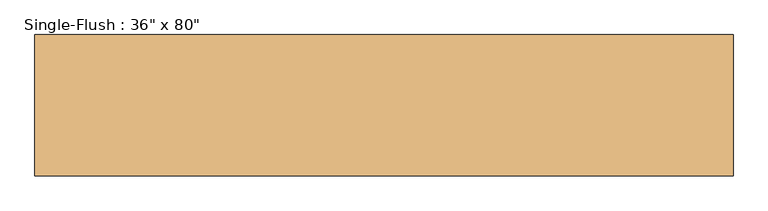
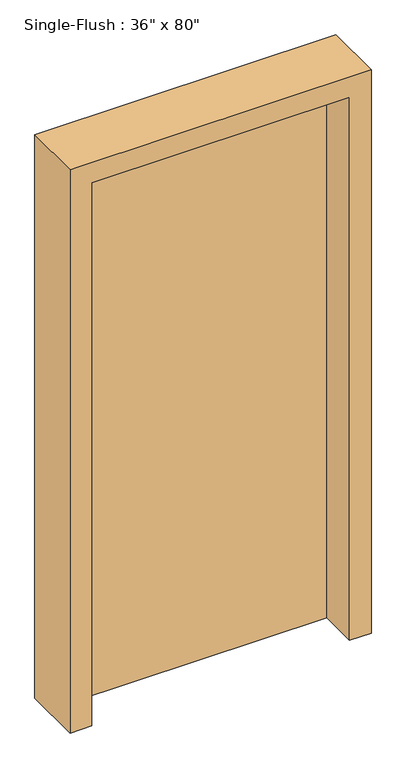
"""IFC4 building model written with IfcOpenShell, lengths in millimetres: door geometry."""

from ifc_helpers import new_model, si_unit, frame, origin, origin_with_axes, place, context, project, spatial, polyline, outline, extrude, source, transform, mapped, element, save


def door_514697dd(model_context):
    return source(origin(), model_context, "Body", "SweptSolid", [
        extrude(outline(polyline([(2108.2, 533.4), (2108.2, -533.4), (0.0, -533.4), (0.0, -457.2), (2032.0, -457.2), (2032.0, 457.2), (0.0, 457.2), (0.0, 533.4), (2108.2, 533.4)])), frame((0.0, -107.95, 0.0), z_axis=(0.0, 1.0, 0.0), x_axis=(0.0, 0.0, 1.0)), (0.0, 0.0, 1.0), 215.9),
        extrude(outline(polyline([(457.2, 31.75), (-457.2, 31.75), (-457.2, 82.55), (457.2, 82.55), (457.2, 31.75)])), origin_with_axes(), (0.0, 0.0, 1.0), 2032.0),
    ])


if __name__ == "__main__":
    model = new_model("IFC4")
    model_context = context("Model", 3, world=origin())
    ifc_project = project(units=[si_unit("LENGTHUNIT", "METRE", prefix="MILLI")], contexts=[model_context])
    site = spatial("IfcSite", under=ifc_project)
    building = spatial("IfcBuilding", under=site)
    placement = place(None, origin())
    door_shape = door_514697dd(model_context)
    element("IfcDoor", 1, ObjectType="Single-Flush : 36\" x 80\"", at=placement, inside=building, context=model_context, shape_type="MappedRepresentation", body=[
        mapped(door_shape, transform((0.0, 0.0, 0.0), x_axis=(1.0, 0.0, 0.0), y_axis=(0.0, 1.0, 0.0), z_axis=(0.0, 0.0, 1.0))),
    ])
    save(model, "model.ifc")

# Revit data of these elements
# Type "Single-Flush : 36\" x 80\""
#   Type Mark = "6"
#   OD_DS_Door_Material = "T.B.D."
#   OD_DS_Door_Type = "SWING"
#   OD_DS_Lockset = "PRIVACY LOCK"
#   Assembly Code = "C1020"
#   Analytic Construction = "<None>"
#   Thickness = 0' - 2"
#   RO Offset = 0' - 0 1/4"
#   Height = 6' - 8"
#   Trim Projection Ext = 0' - 1"
#   Trim Projection Int = 0' - 1"
#   Trim Width = 0' - 3"
#   Width = 3' - 0"
#   Door Material = Closet_1
#   Frame Material = Closet_1
#   Function = (empty or 0)
#   Wall Closure = (empty or 0)
# Element 1 (IfcDoor, "Single-Flush : 36\" x 80\"")
#   Materials on its faces: "Closet_1"
# Materials
#   "Closet_1": class "Paint", colour RGB 200 194 183, transparency 0, Cost = 0
